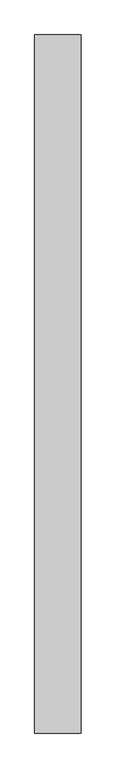
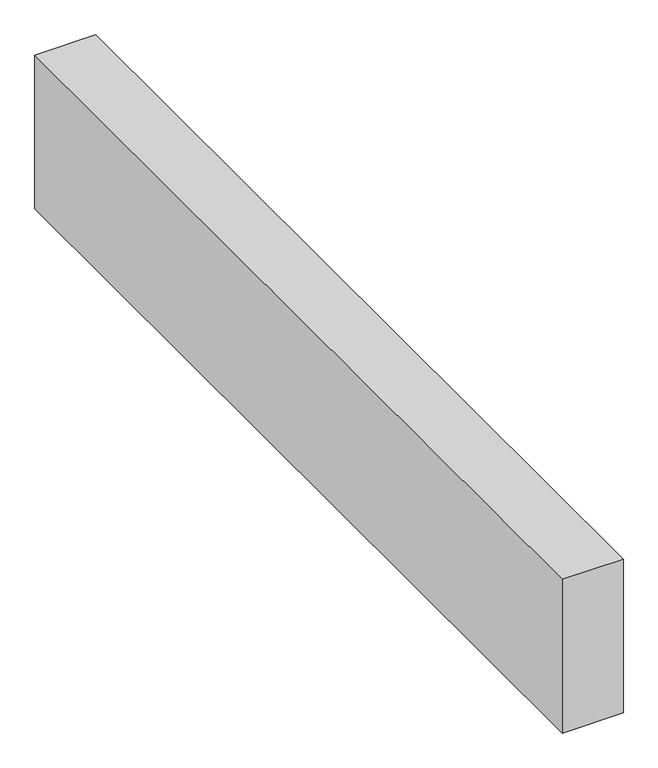
"""IFC4 building model written with IfcOpenShell, lengths in millimetres: proxy geometry, Structure027 331 : Structure027 331."""

import ifcopenshell
import ifcopenshell.guid

model = None  # the IFC model being written
_history = None  # IfcOwnerHistory: only IFC2X3 demands one
_inside = {}  # id of a spatial element -> (the spatial element, [elements in it])
_under = {}  # id of a project, library or spatial element -> (it, [spatial elements below it])
_declared = {}  # id of a project -> (the project, [libraries it declares])
_typed = {}  # id of a type object -> (the type object, [elements of that type])
_made_of = {}  # id of a material, layer set ... -> (it, [elements and type objects made of it])


def new_model(schema):
    """Start an empty IFC model of exactly this schema.

    Asked for "IFC4X3", IfcOpenShell would pick the latest addendum, in which some entities
    have other attributes; the version numbers below select the first issue.
    IFC2X3 requires an IfcOwnerHistory on every rooted entity: one is made here for all.
    """
    global model, _history
    if schema == "IFC4X3":
        model = ifcopenshell.file(schema_version=(4, 3, 0, 0))
    else:
        model = ifcopenshell.file(schema=schema)
    _inside.clear()
    _under.clear()
    _declared.clear()
    _typed.clear()
    _made_of.clear()
    _history = None
    if model.schema == "IFC2X3":
        org = make("IfcOrganization", Name="unknown")
        user = make(
            "IfcPersonAndOrganization",
            ThePerson=make("IfcPerson", FamilyName="unknown"),
            TheOrganization=org,
        )
        app = make(
            "IfcApplication",
            ApplicationDeveloper=org,
            Version="unknown",
            ApplicationFullName="unknown",
            ApplicationIdentifier="unknown",
        )
        _history = make(
            "IfcOwnerHistory",
            OwningUser=user,
            OwningApplication=app,
            ChangeAction="ADDED",
            CreationDate=0,
        )
    return model


def make(cls, **values):
    """One entity of the class cls with the attributes given. An attribute that is None is left unset."""
    return model.create_entity(
        cls, **{name: value for name, value in values.items() if value is not None}
    )


def rooted(cls, **values):
    """An entity with a GlobalId (a new one), such as an element, a storey or a relation."""
    return make(cls, GlobalId=ifcopenshell.guid.new(), OwnerHistory=_history, **values)


def si_unit(unit_type, name, prefix=None):
    """IfcSIUnit, for example si_unit("LENGTHUNIT", "METRE", prefix="MILLI")."""
    return make("IfcSIUnit", UnitType=unit_type, Prefix=prefix, Name=name)


def assignment(units):
    """IfcUnitAssignment: the units of a project."""
    return None if units is None else make("IfcUnitAssignment", Units=units)


def point(xyz):
    """IfcCartesianPoint."""
    return None if xyz is None else make("IfcCartesianPoint", Coordinates=xyz)


def direction(xyz):
    """IfcDirection."""
    return None if xyz is None else make("IfcDirection", DirectionRatios=xyz)


def frame(location, z_axis=None, x_axis=None):
    """IfcAxis2Placement3D, a coordinate frame: its origin and axes. An axis left out is left unset."""
    return make(
        "IfcAxis2Placement3D",
        Location=point(location),
        Axis=direction(z_axis),
        RefDirection=direction(x_axis),
    )


def origin():
    """The frame at (0, 0, 0) with its axes left unset."""
    return frame((0.0, 0.0, 0.0))


def place(relative_to, where):
    """IfcLocalPlacement: puts the frame where relative to a parent placement (None: the world)."""
    return make(
        "IfcLocalPlacement", PlacementRelTo=relative_to, RelativePlacement=where
    )


def context(
    kind, dimensions, precision=None, world=None, true_north=None, identifier=None
):
    """IfcGeometricRepresentationContext, for example the 3D "Model" context."""
    return make(
        "IfcGeometricRepresentationContext",
        ContextIdentifier=identifier,
        ContextType=kind,
        CoordinateSpaceDimension=dimensions,
        Precision=precision,
        WorldCoordinateSystem=world,
        TrueNorth=true_north,
    )


def project(units=None, contexts=None):
    """IfcProject with its units and contexts."""
    return rooted(
        "IfcProject",
        Name="project",
        RepresentationContexts=contexts,
        UnitsInContext=assignment(units),
    )


def spatial(cls, under=None, at=None, **own):
    """A site, building, storey or space (cls), placed at a placement, below another one or the project."""
    s = rooted(cls, ObjectPlacement=at, **own)
    if under is not None:
        _under.setdefault(under.id(), (under, []))[1].append(s)
    return s


def polyline(points):
    """IfcPolyline through the points."""
    return make("IfcPolyline", Points=[point(p) for p in points])


def outline(outer, holes=None, kind="AREA"):
    """IfcArbitraryClosedProfileDef: a profile drawn as a closed curve; with holes, ...WithVoids."""
    if holes is None:
        return make("IfcArbitraryClosedProfileDef", ProfileType=kind, OuterCurve=outer)
    return make(
        "IfcArbitraryProfileDefWithVoids",
        ProfileType=kind,
        OuterCurve=outer,
        InnerCurves=holes,
    )


def extrude(swept, where, along, depth):
    """IfcExtrudedAreaSolid: the profile swept, set in the frame where, extruded along a direction by depth."""
    return make(
        "IfcExtrudedAreaSolid",
        SweptArea=swept,
        Position=where,
        ExtrudedDirection=direction(along),
        Depth=depth,
    )


def shape(context_of_items, identifier, shape_type, items):
    """IfcShapeRepresentation: the items that make up one representation, for example the "Body"."""
    return make(
        "IfcShapeRepresentation",
        ContextOfItems=context_of_items,
        RepresentationIdentifier=identifier,
        RepresentationType=shape_type,
        Items=items,
    )


def source(mapping_origin, context_of_items, identifier, shape_type, items):
    """IfcRepresentationMap: a shape defined once, which mapped items show again and again."""
    return make(
        "IfcRepresentationMap",
        MappingOrigin=mapping_origin,
        MappedRepresentation=shape(context_of_items, identifier, shape_type, items),
    )


def transform(
    local_origin,
    x_axis=None,
    y_axis=None,
    z_axis=None,
    scale=None,
    scale2=None,
    scale3=None,
    uniform=True,
):
    """IfcCartesianTransformationOperator3D, or its non-uniform kind. x_axis, y_axis, z_axis: its Axis1, 2, 3."""
    if uniform:
        return make(
            "IfcCartesianTransformationOperator3D",
            Axis1=direction(x_axis),
            Axis2=direction(y_axis),
            LocalOrigin=point(local_origin),
            Scale=scale,
            Axis3=direction(z_axis),
        )
    return make(
        "IfcCartesianTransformationOperator3DnonUniform",
        Axis1=direction(x_axis),
        Axis2=direction(y_axis),
        LocalOrigin=point(local_origin),
        Scale=scale,
        Axis3=direction(z_axis),
        Scale2=scale2,
        Scale3=scale3,
    )


def mapped(mapping_source, mapping_target):
    """IfcMappedItem: shows the shape of a source again, moved by a transform."""
    return make(
        "IfcMappedItem", MappingSource=mapping_source, MappingTarget=mapping_target
    )


def made_of(thing, what):
    """Note that an element or type object is made of a material, layer set ...; save() writes the relation."""
    if what is not None:
        _made_of.setdefault(what.id(), (what, []))[1].append(thing)
    return thing


def element(
    cls,
    number,
    at=None,
    inside=None,
    cuts=None,
    type_object=None,
    material=None,
    context=None,
    identifier="Body",
    shape_type=None,
    held_by="IfcProductDefinitionShape",
    body=None,
    shapes=None,
    **own,
):
    """One element of the class cls, such as IfcWall. Its Tag is "e" and its number.

    at: its placement. inside: the storey or other place that contains it. cuts: it is an
    opening in that element (IfcRelVoidsElement). A single representation is given by context,
    identifier, shape_type and body (its items); several are given by shapes. held_by: the class
    of the entity that holds the representations. save() writes the other relations.
    """
    e = rooted(cls, Tag="e%d" % number, ObjectPlacement=at, **own)
    if body is not None:
        shapes = [shape(context, identifier, shape_type, body)]
    if shapes is not None:
        e.Representation = make(held_by, Representations=shapes)
    if inside is not None:
        _inside.setdefault(inside.id(), (inside, []))[1].append(e)
    if cuts is not None:
        rooted(
            "IfcRelVoidsElement", RelatingBuildingElement=cuts, RelatedOpeningElement=e
        )
    if type_object is not None:
        _typed.setdefault(type_object.id(), (type_object, []))[1].append(e)
    return made_of(e, material)


def aggregate(whole, parts):
    """IfcRelAggregates: a whole, such as a stair, and the parts it consists of."""
    return rooted("IfcRelAggregates", RelatingObject=whole, RelatedObjects=parts)


def save(model, path):
    """Write the relations noted so far, then the file.

    IfcRelAggregates (storeys below a building ...), IfcRelContainedInSpatialStructure (elements
    in a storey), IfcRelDefinesByType, IfcRelAssociatesMaterial and IfcRelDeclares: one each for
    every whole, place, type object, material and project.
    """
    for whole, parts in _under.values():
        aggregate(whole, parts)
    for where, things in _inside.values():
        rooted(
            "IfcRelContainedInSpatialStructure",
            RelatedElements=things,
            RelatingStructure=where,
        )
    for kind, things in _typed.values():
        rooted("IfcRelDefinesByType", RelatedObjects=things, RelatingType=kind)
    for what, things in _made_of.values():
        rooted("IfcRelAssociatesMaterial", RelatedObjects=things, RelatingMaterial=what)
    for by, libraries in _declared.values():
        rooted("IfcRelDeclares", RelatingContext=by, RelatedDefinitions=libraries)
    model.write(path)


def generic_models_7d935cd3(model_context):
    return source(origin(), model_context, "Body", "SweptSolid", [
        extrude(outline(polyline([(-9755.5737014, 7982.1531721), (-9888.9237014, 7982.1531721), (-9888.9237014, 9982.1531721), (-9755.5737014, 9982.1531721), (-9755.5737014, 7982.1531721)])), frame((0.0, 0.0, 39579.2960083), z_axis=(0.0, 0.0, 1.0), x_axis=(1.0, 0.0, 0.0)), (0.0, 0.0, 1.0), 355.6),
    ])


if __name__ == "__main__":
    model = new_model("IFC4")
    model_context = context("Model", 3, world=origin())
    ifc_project = project(units=[si_unit("LENGTHUNIT", "METRE", prefix="MILLI")], contexts=[model_context])
    site = spatial("IfcSite", under=ifc_project)
    building = spatial("IfcBuilding", under=site)
    placement = place(None, origin())
    generic_models_shape = generic_models_7d935cd3(model_context)
    element("IfcBuildingElementProxy", 1, Name="Structure027 331 : Structure027 331", ObjectType="Structure027 331 : Structure027 331", at=placement, inside=building, context=model_context, shape_type="MappedRepresentation", body=[
        mapped(generic_models_shape, transform((0.0, 0.0, 0.0), x_axis=(1.0, 0.0, 0.0), y_axis=(0.0, 1.0, 0.0), z_axis=(0.0, 0.0, 1.0))),
    ])
    save(model, "model.ifc")

# Revit data of these elements
# Type "Structure027 331 : Structure027 331"
#   NameOverride = "Structure027"
# Element 1 (IfcBuildingElementProxy, "Structure027 331 : Structure027 331")
#   Materials on its faces: "STRUCTURAL MEMBER (SEE STRUCTURAL DWGS)"
# Materials
#   "STRUCTURAL MEMBER (SEE STRUCTURAL DWGS)": class "Unassigned", colour RGB 176 134 95, transparency 0, Cost = 0
